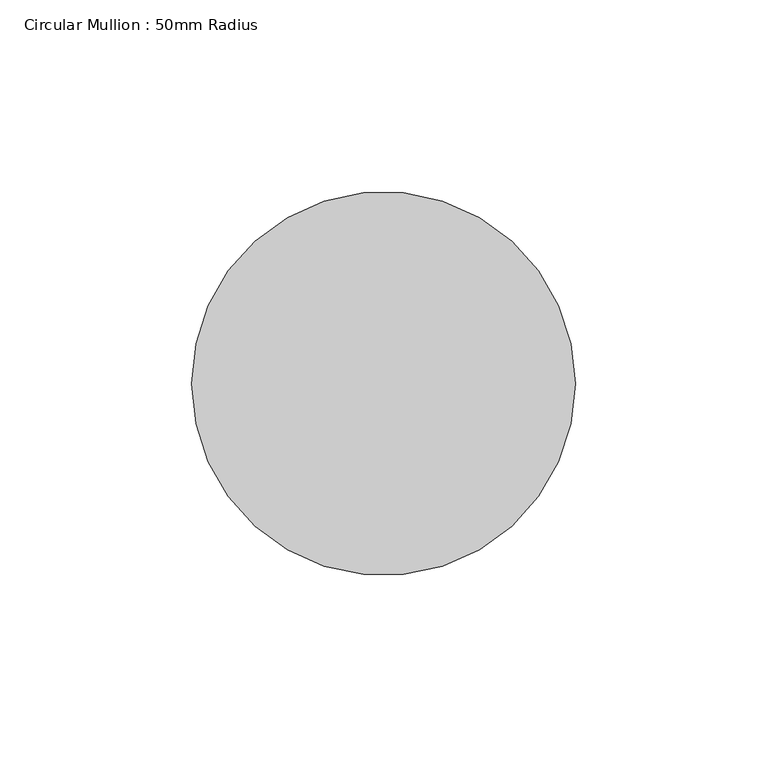
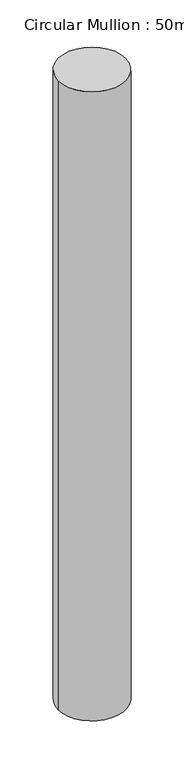
"""IFC4 building model written with IfcOpenShell, lengths in millimetres: member geometry, Circular Mullion : 50mm Radius."""

import ifcopenshell
import ifcopenshell.guid

model = None  # the IFC model being written
_history = None  # IfcOwnerHistory: only IFC2X3 demands one
_inside = {}  # id of a spatial element -> (the spatial element, [elements in it])
_under = {}  # id of a project, library or spatial element -> (it, [spatial elements below it])
_declared = {}  # id of a project -> (the project, [libraries it declares])
_typed = {}  # id of a type object -> (the type object, [elements of that type])
_made_of = {}  # id of a material, layer set ... -> (it, [elements and type objects made of it])


def new_model(schema):
    """Start an empty IFC model of exactly this schema.

    Asked for "IFC4X3", IfcOpenShell would pick the latest addendum, in which some entities
    have other attributes; the version numbers below select the first issue.
    IFC2X3 requires an IfcOwnerHistory on every rooted entity: one is made here for all.
    """
    global model, _history
    if schema == "IFC4X3":
        model = ifcopenshell.file(schema_version=(4, 3, 0, 0))
    else:
        model = ifcopenshell.file(schema=schema)
    _inside.clear()
    _under.clear()
    _declared.clear()
    _typed.clear()
    _made_of.clear()
    _history = None
    if model.schema == "IFC2X3":
        org = make("IfcOrganization", Name="unknown")
        user = make(
            "IfcPersonAndOrganization",
            ThePerson=make("IfcPerson", FamilyName="unknown"),
            TheOrganization=org,
        )
        app = make(
            "IfcApplication",
            ApplicationDeveloper=org,
            Version="unknown",
            ApplicationFullName="unknown",
            ApplicationIdentifier="unknown",
        )
        _history = make(
            "IfcOwnerHistory",
            OwningUser=user,
            OwningApplication=app,
            ChangeAction="ADDED",
            CreationDate=0,
        )
    return model


def make(cls, **values):
    """One entity of the class cls with the attributes given. An attribute that is None is left unset."""
    return model.create_entity(
        cls, **{name: value for name, value in values.items() if value is not None}
    )


def rooted(cls, **values):
    """An entity with a GlobalId (a new one), such as an element, a storey or a relation."""
    return make(cls, GlobalId=ifcopenshell.guid.new(), OwnerHistory=_history, **values)


def si_unit(unit_type, name, prefix=None):
    """IfcSIUnit, for example si_unit("LENGTHUNIT", "METRE", prefix="MILLI")."""
    return make("IfcSIUnit", UnitType=unit_type, Prefix=prefix, Name=name)


def assignment(units):
    """IfcUnitAssignment: the units of a project."""
    return None if units is None else make("IfcUnitAssignment", Units=units)


def point(xyz):
    """IfcCartesianPoint."""
    return None if xyz is None else make("IfcCartesianPoint", Coordinates=xyz)


def direction(xyz):
    """IfcDirection."""
    return None if xyz is None else make("IfcDirection", DirectionRatios=xyz)


def frame(location, z_axis=None, x_axis=None):
    """IfcAxis2Placement3D, a coordinate frame: its origin and axes. An axis left out is left unset."""
    return make(
        "IfcAxis2Placement3D",
        Location=point(location),
        Axis=direction(z_axis),
        RefDirection=direction(x_axis),
    )


def frame_2d(location, x_axis=None):
    """IfcAxis2Placement2D, a coordinate frame in the plane: its origin and x axis."""
    return make(
        "IfcAxis2Placement2D", Location=point(location), RefDirection=direction(x_axis)
    )


def origin():
    """The frame at (0, 0, 0) with its axes left unset."""
    return frame((0.0, 0.0, 0.0))


def origin_2d():
    """The frame at (0, 0) in the plane with its x axis left unset."""
    return frame_2d((0.0, 0.0))


def place(relative_to, where):
    """IfcLocalPlacement: puts the frame where relative to a parent placement (None: the world)."""
    return make(
        "IfcLocalPlacement", PlacementRelTo=relative_to, RelativePlacement=where
    )


def context(
    kind, dimensions, precision=None, world=None, true_north=None, identifier=None
):
    """IfcGeometricRepresentationContext, for example the 3D "Model" context."""
    return make(
        "IfcGeometricRepresentationContext",
        ContextIdentifier=identifier,
        ContextType=kind,
        CoordinateSpaceDimension=dimensions,
        Precision=precision,
        WorldCoordinateSystem=world,
        TrueNorth=true_north,
    )


def project(units=None, contexts=None):
    """IfcProject with its units and contexts."""
    return rooted(
        "IfcProject",
        Name="project",
        RepresentationContexts=contexts,
        UnitsInContext=assignment(units),
    )


def spatial(cls, under=None, at=None, **own):
    """A site, building, storey or space (cls), placed at a placement, below another one or the project."""
    s = rooted(cls, ObjectPlacement=at, **own)
    if under is not None:
        _under.setdefault(under.id(), (under, []))[1].append(s)
    return s


def circle_curve(where, radius):
    """IfcCircle in the frame where."""
    return make("IfcCircle", Position=where, Radius=radius)


def trimmed(basis, trim1, trim2, sense, master):
    """IfcTrimmedCurve: the piece of a basis curve between two trims."""
    return make(
        "IfcTrimmedCurve",
        BasisCurve=basis,
        Trim1=trim1,
        Trim2=trim2,
        SenseAgreement=sense,
        MasterRepresentation=master,
    )


def segment(curve, same_sense, transition):
    """IfcCompositeCurveSegment."""
    return make(
        "IfcCompositeCurveSegment",
        Transition=transition,
        SameSense=same_sense,
        ParentCurve=curve,
    )


def composite_curve(segments, self_intersect=None):
    """IfcCompositeCurve: segments joined end to end."""
    return make("IfcCompositeCurve", Segments=segments, SelfIntersect=self_intersect)


def outline(outer, holes=None, kind="AREA"):
    """IfcArbitraryClosedProfileDef: a profile drawn as a closed curve; with holes, ...WithVoids."""
    if holes is None:
        return make("IfcArbitraryClosedProfileDef", ProfileType=kind, OuterCurve=outer)
    return make(
        "IfcArbitraryProfileDefWithVoids",
        ProfileType=kind,
        OuterCurve=outer,
        InnerCurves=holes,
    )


def extrude(swept, where, along, depth):
    """IfcExtrudedAreaSolid: the profile swept, set in the frame where, extruded along a direction by depth."""
    return make(
        "IfcExtrudedAreaSolid",
        SweptArea=swept,
        Position=where,
        ExtrudedDirection=direction(along),
        Depth=depth,
    )


def shape(context_of_items, identifier, shape_type, items):
    """IfcShapeRepresentation: the items that make up one representation, for example the "Body"."""
    return make(
        "IfcShapeRepresentation",
        ContextOfItems=context_of_items,
        RepresentationIdentifier=identifier,
        RepresentationType=shape_type,
        Items=items,
    )


def source(mapping_origin, context_of_items, identifier, shape_type, items):
    """IfcRepresentationMap: a shape defined once, which mapped items show again and again."""
    return make(
        "IfcRepresentationMap",
        MappingOrigin=mapping_origin,
        MappedRepresentation=shape(context_of_items, identifier, shape_type, items),
    )


def transform(
    local_origin,
    x_axis=None,
    y_axis=None,
    z_axis=None,
    scale=None,
    scale2=None,
    scale3=None,
    uniform=True,
):
    """IfcCartesianTransformationOperator3D, or its non-uniform kind. x_axis, y_axis, z_axis: its Axis1, 2, 3."""
    if uniform:
        return make(
            "IfcCartesianTransformationOperator3D",
            Axis1=direction(x_axis),
            Axis2=direction(y_axis),
            LocalOrigin=point(local_origin),
            Scale=scale,
            Axis3=direction(z_axis),
        )
    return make(
        "IfcCartesianTransformationOperator3DnonUniform",
        Axis1=direction(x_axis),
        Axis2=direction(y_axis),
        LocalOrigin=point(local_origin),
        Scale=scale,
        Axis3=direction(z_axis),
        Scale2=scale2,
        Scale3=scale3,
    )


def mapped(mapping_source, mapping_target):
    """IfcMappedItem: shows the shape of a source again, moved by a transform."""
    return make(
        "IfcMappedItem", MappingSource=mapping_source, MappingTarget=mapping_target
    )


def made_of(thing, what):
    """Note that an element or type object is made of a material, layer set ...; save() writes the relation."""
    if what is not None:
        _made_of.setdefault(what.id(), (what, []))[1].append(thing)
    return thing


def element(
    cls,
    number,
    at=None,
    inside=None,
    cuts=None,
    type_object=None,
    material=None,
    context=None,
    identifier="Body",
    shape_type=None,
    held_by="IfcProductDefinitionShape",
    body=None,
    shapes=None,
    **own,
):
    """One element of the class cls, such as IfcWall. Its Tag is "e" and its number.

    at: its placement. inside: the storey or other place that contains it. cuts: it is an
    opening in that element (IfcRelVoidsElement). A single representation is given by context,
    identifier, shape_type and body (its items); several are given by shapes. held_by: the class
    of the entity that holds the representations. save() writes the other relations.
    """
    e = rooted(cls, Tag="e%d" % number, ObjectPlacement=at, **own)
    if body is not None:
        shapes = [shape(context, identifier, shape_type, body)]
    if shapes is not None:
        e.Representation = make(held_by, Representations=shapes)
    if inside is not None:
        _inside.setdefault(inside.id(), (inside, []))[1].append(e)
    if cuts is not None:
        rooted(
            "IfcRelVoidsElement", RelatingBuildingElement=cuts, RelatedOpeningElement=e
        )
    if type_object is not None:
        _typed.setdefault(type_object.id(), (type_object, []))[1].append(e)
    return made_of(e, material)


def aggregate(whole, parts):
    """IfcRelAggregates: a whole, such as a stair, and the parts it consists of."""
    return rooted("IfcRelAggregates", RelatingObject=whole, RelatedObjects=parts)


def save(model, path):
    """Write the relations noted so far, then the file.

    IfcRelAggregates (storeys below a building ...), IfcRelContainedInSpatialStructure (elements
    in a storey), IfcRelDefinesByType, IfcRelAssociatesMaterial and IfcRelDeclares: one each for
    every whole, place, type object, material and project.
    """
    for whole, parts in _under.values():
        aggregate(whole, parts)
    for where, things in _inside.values():
        rooted(
            "IfcRelContainedInSpatialStructure",
            RelatedElements=things,
            RelatingStructure=where,
        )
    for kind, things in _typed.values():
        rooted("IfcRelDefinesByType", RelatedObjects=things, RelatingType=kind)
    for what, things in _made_of.values():
        rooted("IfcRelAssociatesMaterial", RelatedObjects=things, RelatingMaterial=what)
    for by, libraries in _declared.values():
        rooted("IfcRelDeclares", RelatingContext=by, RelatedDefinitions=libraries)
    model.write(path)


def circular_mullion_50mm_radius_f7d9cbfb(model_context):
    return source(origin(), model_context, "Body", "SweptSolid", [
        extrude(outline(composite_curve([segment(trimmed(circle_curve(origin_2d(), 50.0), [point((50.0, 0.0))], [point((-50.0, 0.0))], False, "CARTESIAN"), True, "CONTINUOUS"), segment(trimmed(circle_curve(origin_2d(), 50.0), [point((-50.0, 0.0))], [point((50.0, 0.0))], False, "CARTESIAN"), True, "CONTINUOUS")], self_intersect=False)), frame((0.0, 0.0, -985.7302805), z_axis=(0.0, 0.0, 1.0), x_axis=(1.0, 0.0, 0.0)), (0.0, 0.0, 1.0), 985.7302805),
    ])


if __name__ == "__main__":
    model = new_model("IFC4")
    model_context = context("Model", 3, world=origin())
    ifc_project = project(units=[si_unit("LENGTHUNIT", "METRE", prefix="MILLI")], contexts=[model_context])
    site = spatial("IfcSite", under=ifc_project)
    building = spatial("IfcBuilding", under=site)
    placement = place(None, origin())
    circular_mullion_50mm_radius_shape = circular_mullion_50mm_radius_f7d9cbfb(model_context)
    element("IfcMember", 1, ObjectType="Circular Mullion : 50mm Radius", at=placement, inside=building, context=model_context, shape_type="MappedRepresentation", body=[
        mapped(circular_mullion_50mm_radius_shape, transform((0.0, 0.0, 0.0), x_axis=(1.0, 0.0, 0.0), y_axis=(0.0, 1.0, 0.0), z_axis=(0.0, 0.0, 1.0))),
    ])
    save(model, "model.ifc")

# Revit data of these elements
# Type "Circular Mullion : 50mm Radius"
#   built-in parameter 1007350 = 0.164042 (stored number, unit not read)
# Element 1 (IfcMember, "Circular Mullion : 50mm Radius")
#   Materials on its faces: "Aluminium"
# Materials
#   "Aluminium": class "Metal", colour RGB 247 247 247, transparency 0, Description = "Aluminium 6061", Cost = 0
